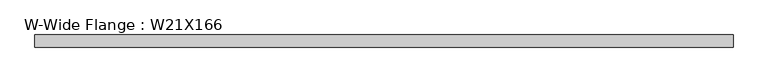
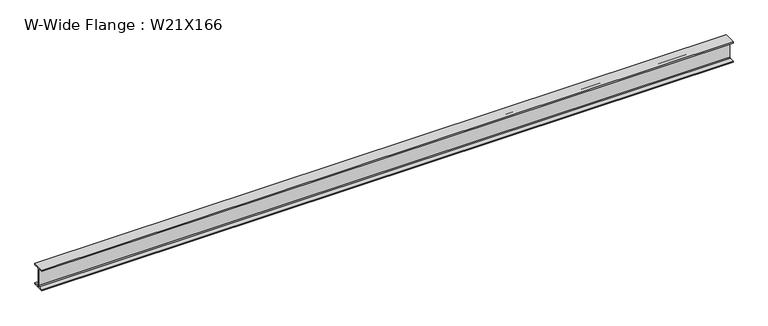
"""IFC4 building model written with IfcOpenShell, lengths in millimetres: beam geometry, W-Wide Flange : W21X166."""

from ifc_helpers import new_model, si_unit, point, frame, frame_2d, origin, place, context, project, spatial, polyline, circle_curve, trimmed, segment, composite_curve, outline, extrude, source, transform, mapped, element, save


def w_wide_flange_w21x166_f950f755(model_context):
    return source(origin(), model_context, "Body", "SweptSolid", [
        extrude(outline(composite_curve([segment(polyline([(157.48, -251.206), (157.48, -285.75), (-157.48, -285.75), (-157.48, -251.206), (-32.131, -251.206)]), True, "CONTINUOUS"), segment(trimmed(circle_curve(frame_2d((-32.131, -228.6)), 22.606), [point((-32.131, -251.206))], [point((-9.525, -228.6))], True, "CARTESIAN"), True, "CONTINUOUS"), segment(polyline([(-9.525, -228.6), (-9.525, 228.6)]), True, "CONTINUOUS"), segment(trimmed(circle_curve(frame_2d((-32.131, 228.6)), 22.606), [point((-9.525, 228.6))], [point((-32.131, 251.206))], True, "CARTESIAN"), True, "CONTINUOUS"), segment(polyline([(-32.131, 251.206), (-157.48, 251.206), (-157.48, 285.75), (157.48, 285.75), (157.48, 251.206), (32.131, 251.206)]), True, "CONTINUOUS"), segment(trimmed(circle_curve(frame_2d((32.131, 228.6)), 22.606), [point((32.131, 251.206))], [point((9.525, 228.6))], True, "CARTESIAN"), True, "CONTINUOUS"), segment(polyline([(9.525, 228.6), (9.525, -228.6)]), True, "CONTINUOUS"), segment(trimmed(circle_curve(frame_2d((32.131, -228.6)), 22.606), [point((9.525, -228.6))], [point((32.131, -251.206))], True, "CARTESIAN"), True, "CONTINUOUS"), segment(polyline([(32.131, -251.206), (157.48, -251.206)]), True, "CONTINUOUS")], self_intersect=False)), frame((-9151.4273842, 0.0, 0.0), z_axis=(1.0, 0.0, 0.0), x_axis=(0.0, 1.0, 0.0)), (0.0, 0.0, 1.0), 18150.0379668),
    ])


if __name__ == "__main__":
    model = new_model("IFC4")
    model_context = context("Model", 3, world=origin())
    ifc_project = project(units=[si_unit("LENGTHUNIT", "METRE", prefix="MILLI")], contexts=[model_context])
    site = spatial("IfcSite", under=ifc_project)
    building = spatial("IfcBuilding", under=site)
    placement = place(None, origin())
    w_wide_flange_w21x166_shape = w_wide_flange_w21x166_f950f755(model_context)
    element("IfcBeam", 1, ObjectType="W-Wide Flange : W21X166", at=placement, inside=building, context=model_context, shape_type="MappedRepresentation", body=[
        mapped(w_wide_flange_w21x166_shape, transform((0.0, 0.0, 0.0), x_axis=(1.0, 0.0, 0.0), y_axis=(0.0, 1.0, 0.0), z_axis=(0.0, 0.0, 1.0))),
    ])
    save(model, "model.ifc")

# Revit data of these elements
# Type "W-Wide Flange : W21X166"
#   Assembly Code = "B10"
#   W = 166
#   Length [instance default] = 5' - 0"
#   bf = 1' - 0.4"
#   d = 1' - 10 1/2"
#   k = 0' - 2 1/4"
#   k2 = 0' - 0.89"
#   tf = 0' - 1.36"
#   tw = 0' - 0 3/4"
#   A = 0.338889 SF
#   Structural Material [instance default] = Steel ASTM A992
# Element 1 (IfcBeam, "W-Wide Flange : W21X166")
#   Structural Material = Steel
#   Materials on its faces: "Steel"
# Materials
#   "Steel ASTM A992": class "Metal", colour RGB 199 199 199, transparency 0, Description = "Structural steel 50ksi", Cost = 0
#   "Steel": class "Metal", colour RGB 118 118 114, transparency 0, Description = "Steel, mill finish", Cost = 0
